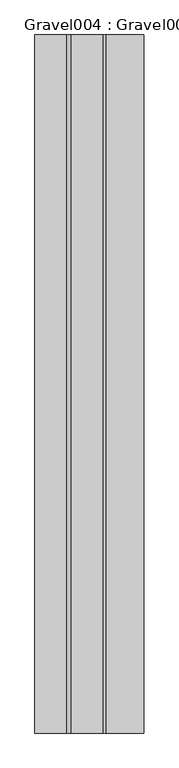
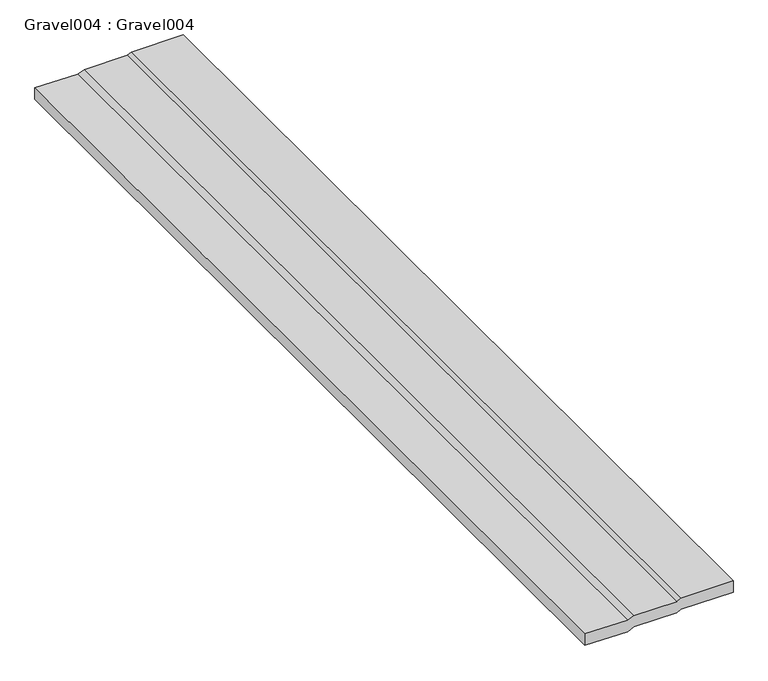
"""IFC4 building model written with IfcOpenShell, lengths in millimetres: proxy geometry, Gravel004 : Gravel004."""

from ifc_helpers import new_model, si_unit, frame, origin, place, context, project, spatial, polyline, outline, extrude, source, transform, mapped, element, save


def gravel004_gravel004_468a0762(model_context):
    return source(origin(), model_context, "Body", "SweptSolid", [
        extrude(outline(polyline([(40274.2359464, -4497.235977), (40274.2359464, -4387.7364653), (40298.9742277, -4387.7364653), (40298.9742277, -4497.235977), (40294.6929777, -4505.9464262), (40294.6929777, -4596.5333403), (40288.9655157, -4609.3779796), (40290.6109464, -4699.8063764), (40265.8726651, -4699.8063764), (40264.2272344, -4609.3779796), (40269.9546964, -4596.5333403), (40269.9546964, -4505.9464262), (40274.2359464, -4497.235977)])), frame((0.0, -1052.6406573, 0.0), z_axis=(0.0, 1.0, 0.0), x_axis=(0.0, 0.0, 1.0)), (0.0, 0.0, 1.0), 2000.0),
    ])


if __name__ == "__main__":
    model = new_model("IFC4")
    model_context = context("Model", 3, world=origin())
    ifc_project = project(units=[si_unit("LENGTHUNIT", "METRE", prefix="MILLI")], contexts=[model_context])
    site = spatial("IfcSite", under=ifc_project)
    building = spatial("IfcBuilding", under=site)
    placement = place(None, origin())
    gravel004_gravel004_shape = gravel004_gravel004_468a0762(model_context)
    element("IfcBuildingElementProxy", 1, Name="Gravel004 : Gravel004", ObjectType="Gravel004 : Gravel004", at=placement, inside=building, context=model_context, shape_type="MappedRepresentation", body=[
        mapped(gravel004_gravel004_shape, transform((0.0, 0.0, 0.0), x_axis=(1.0, 0.0, 0.0), y_axis=(0.0, 1.0, 0.0), z_axis=(0.0, 0.0, 1.0))),
    ])
    save(model, "model.ifc")

# Revit data of these elements
# Type "Gravel004 : Gravel004"
#   NameOverride = "Gravel004"
# Element 1 (IfcBuildingElementProxy, "Gravel004 : Gravel004")
#   Materials on its faces: "GRAVEL BALLAST"
# Materials
#   "GRAVEL BALLAST": class "Unassigned", colour RGB 128 128 128, transparency 0, Cost = 0
